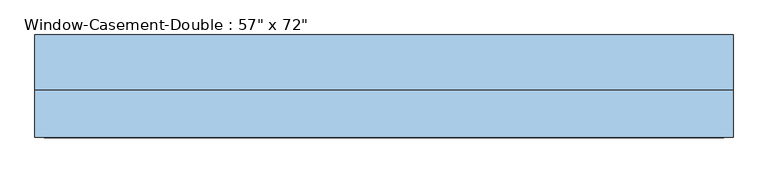
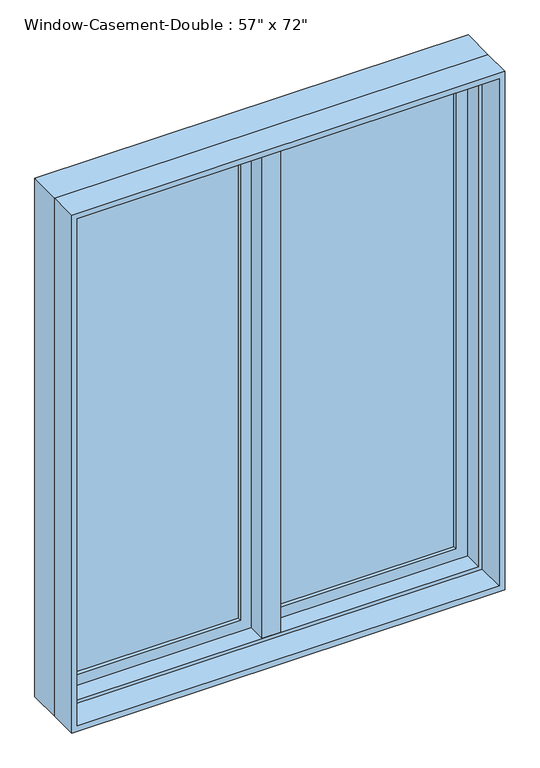
"""IFC4 building model written with IfcOpenShell, lengths in millimetres: window geometry."""

from ifc_helpers import new_model, si_unit, frame, origin, place, context, project, spatial, polyline, outline, extrude, faceted_brep, source, transform, mapped, element, save


def window_696a771e(model_context):
    return source(origin(), model_context, "Body", "SolidModel", [
        faceted_brep([(9.525, 115.8875, 2730.5), (-9.525, 115.8875, 2730.5), (-9.525, 65.0875, 2730.5), (9.525, 65.0875, 2730.5), (9.525, 115.8875, 927.1), (9.525, 65.0875, 927.1), (-9.525, 65.0875, 927.1), (-9.525, 115.8875, 927.1), (-9.525, 65.0875, 946.15), (-9.525, 65.0875, 2711.45), (-30.1625, 65.0875, 946.15), (-30.1625, 65.0875, 2711.45), (-30.1625, 1.5875, 946.15), (-30.1625, 1.5875, 2711.45), (30.1625, 1.5875, 946.15), (30.1625, 1.5875, 2711.45), (30.1625, 65.0875, 946.15), (30.1625, 65.0875, 2711.45), (9.525, 65.0875, 946.15), (9.525, 65.0875, 2711.45)], [[[0, 1, 2, 3]], [[4, 5, 6, 7]], [[1, 0, 4, 7]], [[2, 1, 7, 6, 8, 9]], [[9, 8, 10, 11]], [[11, 10, 12, 13]], [[13, 12, 14, 15]], [[15, 14, 16, 17]], [[17, 16, 18, 19]], [[0, 3, 19, 18, 5, 4]], [[18, 8, 6, 5]], [[9, 19, 3, 2]], [[8, 18, 16, 14, 12, 10]], [[19, 9, 11, 13, 15, 17]]]),
        extrude(outline(polyline([(-66.675, 96.8375), (-66.675, 90.4875), (-654.05, 90.4875), (-654.05, 96.8375), (-66.675, 96.8375)])), frame((0.0, 0.0, 984.25), z_axis=(0.0, 0.0, 1.0), x_axis=(1.0, 0.0, 0.0)), (0.0, 0.0, 1.0), 1689.1),
        extrude(outline(polyline([(-654.05, 77.7875), (-654.05, 84.1375), (-66.675, 84.1375), (-66.675, 77.7875), (-654.05, 77.7875)])), frame((0.0, 0.0, 984.25), z_axis=(0.0, 0.0, 1.0), x_axis=(1.0, 0.0, 0.0)), (0.0, 0.0, 1.0), 1689.1),
        extrude(outline(polyline([(654.05, 96.8375), (654.05, 90.4875), (66.675, 90.4875), (66.675, 96.8375), (654.05, 96.8375)])), frame((0.0, 0.0, 984.25), z_axis=(0.0, 0.0, 1.0), x_axis=(1.0, 0.0, 0.0)), (0.0, 0.0, 1.0), 1689.1),
        extrude(outline(polyline([(66.675, 77.7875), (66.675, 84.1375), (654.05, 84.1375), (654.05, 77.7875), (66.675, 77.7875)])), frame((0.0, 0.0, 984.25), z_axis=(0.0, 0.0, 1.0), x_axis=(1.0, 0.0, 0.0)), (0.0, 0.0, 1.0), 1689.1),
        extrude(outline(polyline([(2730.5, -711.2), (927.1, -711.2), (927.1, -9.525), (2730.5, -9.525), (2730.5, -711.2)]), holes=[polyline([(2673.35, -66.675), (984.25, -66.675), (984.25, -654.05), (2673.35, -654.05), (2673.35, -66.675)])]), frame((0.0, 65.0875, 0.0), z_axis=(0.0, 1.0, 0.0), x_axis=(0.0, 0.0, 1.0)), (0.0, 0.0, 1.0), 44.45),
        extrude(outline(polyline([(927.1, 711.2), (2730.5, 711.2), (2730.5, 9.525), (927.1, 9.525), (927.1, 711.2)]), holes=[polyline([(984.25, 66.675), (2673.35, 66.675), (2673.35, 654.05), (984.25, 654.05), (984.25, 66.675)])]), frame((0.0, 65.0875, 0.0), z_axis=(0.0, 1.0, 0.0), x_axis=(0.0, 0.0, 1.0)), (0.0, 0.0, 1.0), 44.45),
        extrude(outline(polyline([(2743.2, -723.9), (914.4, -723.9), (914.4, 723.9), (2743.2, 723.9), (2743.2, -723.9)]), holes=[polyline([(2724.15, 704.85), (933.45, 704.85), (933.45, -704.85), (2724.15, -704.85), (2724.15, 704.85)])]), frame((0.0, -96.8375, 0.0), z_axis=(0.0, 1.0, 0.0), x_axis=(0.0, 0.0, 1.0)), (0.0, 0.0, 1.0), 98.425),
        faceted_brep([(692.15, 65.0875, 2711.45), (692.15, 1.5875, 2711.45), (-692.15, 1.5875, 2711.45), (-692.15, 65.0875, 2711.45), (711.2, 115.8875, 2730.5), (711.2, 65.0875, 2730.5), (-711.2, 65.0875, 2730.5), (-711.2, 115.8875, 2730.5), (723.9, 1.5875, 2743.2), (723.9, 115.8875, 2743.2), (-723.9, 115.8875, 2743.2), (-723.9, 1.5875, 2743.2), (-692.15, 1.5875, 946.15), (-692.15, 65.0875, 946.15), (-711.2, 65.0875, 927.1), (-711.2, 115.8875, 927.1), (-723.9, 115.8875, 914.4), (-723.9, 1.5875, 914.4), (692.15, 1.5875, 946.15), (692.15, 65.0875, 946.15), (711.2, 65.0875, 927.1), (711.2, 115.8875, 927.1), (723.9, 115.8875, 914.4), (723.9, 1.5875, 914.4)], [[[0, 1, 2, 3]], [[4, 5, 6, 7]], [[8, 9, 10, 11]], [[3, 2, 12, 13]], [[7, 6, 14, 15]], [[11, 10, 16, 17]], [[13, 12, 18, 19]], [[15, 14, 20, 21]], [[17, 16, 22, 23]], [[11, 17, 23, 8], [1, 18, 12, 2]], [[19, 18, 1, 0]], [[5, 20, 14, 6], [3, 13, 19, 0]], [[21, 20, 5, 4]], [[23, 22, 9, 8]], [[9, 22, 16, 10], [7, 15, 21, 4]]]),
    ])


if __name__ == "__main__":
    model = new_model("IFC4")
    model_context = context("Model", 3, world=origin())
    ifc_project = project(units=[si_unit("LENGTHUNIT", "METRE", prefix="MILLI")], contexts=[model_context])
    site = spatial("IfcSite", under=ifc_project)
    building = spatial("IfcBuilding", under=site)
    placement = place(None, origin())
    window_shape = window_696a771e(model_context)
    element("IfcWindow", 1, ObjectType="Window-Casement-Double : 57\" x 72\"", at=placement, inside=building, context=model_context, shape_type="MappedRepresentation", body=[
        mapped(window_shape, transform((0.0, 0.0, 0.0), x_axis=(1.0, 0.0, 0.0), y_axis=(0.0, 1.0, 0.0), z_axis=(0.0, 0.0, 1.0))),
    ])
    save(model, "model.ifc")

# Revit data of these elements
# Type "Window-Casement-Double : 57\" x 72\""
#   Type Mark = "62"
#   Fire Rating = "0.5h"
#   Assembly Code = "B2020100"
#   Analytic Construction = "Double glazing - domestic"
#   Frame Extension [instance default] = 0' - 0 1/4"
#   Window Inset [instance default] = 0' - 0"
#   Wall Thickness [instance default] = 0' - 6"
#   Interior Wall Closure [instance default] = 0' - 2 1/4"
#   Half Width = 2' - 4 1/2"
#   Visual Light Transmittance = 0.81
#   Thermal Resistance (R) = 1.8146 (h·ft²·°F)/BTU
#   Solar Heat Gain Coefficient = 0.76
#   Rough Width = 4' - 9 1/2"
#   Rough Height = 6' - 0 1/2"
#   Height = 6' - 0"
#   Heat Transfer Coefficient (U) = 0.5511 BTU/(h·ft²·°F)
#   Exterior Wall Closure [instance default] = 0' - 1 1/4"
#   Extension Jamb [instance default] = 0' - 2 1/4"
#   Default Sill Height = 3' - 0"
#   Width = 4' - 9"
#   Define Thermal Properties by = 0
#   Muntin Visibility = yes
#   Interior Trim Visibility [instance default] = yes
#   Exterior Trim Visibility [instance default] = yes
#   Extension Jamb Visibility [instance default] = yes
#   Interior Trim Material = Wood - Stained
#   Muntin Pattern = Muntin Pattern_2x2 : Muntin Pattern_2x2
#   Interior Trim = Trim-Window-Interior-Flat : Picture Frame
#   Interior Frame Material = Wood - Stained
#   Glass Panel Material = Glass
#   Exterior Trim Material = Clad - White
#   Exterior Trim = Trim-Window-Exterior-Flat : with Sill
#   Exterior Frame Material = Clad - White
#   Wall Closure = (empty or 0)
# Element 1 (IfcWindow, "Window-Casement-Double : 57\" x 72\"")
#   Wall Thickness = 0' - 7 5/8"
#   Extension Jamb = 0' - 3 7/8"
#   Materials on its faces: "Wood - Stained", "Glass", "Clad - White"
# Materials
#   "Wood - Stained": class "Wood", colour RGB 224 178 126, transparency 0, Cost = 0
#   "Glass": class "Glass", colour RGB 236 240 239, transparency 0.5, Description = "Soda Lime Glass", Cost = 0
#   "Clad - White": class "Wood", colour RGB 216 216 204, transparency 0, Cost = 0
